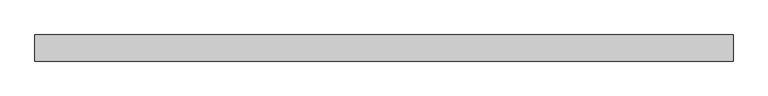
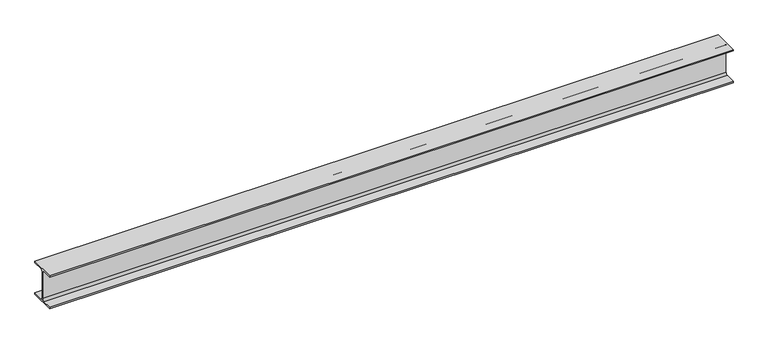
"""IFC4 building model written with IfcOpenShell, lengths in millimetres: beam geometry, 0912_Steel Framing_H-KSD3502 : H_SB_ASB_H-340x250x9x14."""

from ifc_helpers import new_model, si_unit, point, frame, frame_2d, origin, place, context, project, spatial, polyline, circle_curve, trimmed, segment, composite_curve, outline, extrude, source, transform, mapped, element, save


def beam_bd123048(model_context):
    return source(origin(), model_context, "Body", "SweptSolid", [
        extrude(outline(composite_curve([segment(polyline([(125.0, -156.0), (125.0, -170.0), (-125.0, -170.0), (-125.0, -156.0), (-24.5, -156.0)]), True, "CONTINUOUS"), segment(trimmed(circle_curve(frame_2d((-24.5, -136.0)), 20.0), [point((-24.5, -156.0))], [point((-4.5, -136.0))], True, "CARTESIAN"), True, "CONTINUOUS"), segment(polyline([(-4.5, -136.0), (-4.5, 136.0)]), True, "CONTINUOUS"), segment(trimmed(circle_curve(frame_2d((-24.5, 136.0)), 20.0), [point((-4.5, 136.0))], [point((-24.5, 156.0))], True, "CARTESIAN"), True, "CONTINUOUS"), segment(polyline([(-24.5, 156.0), (-125.0, 156.0), (-125.0, 170.0), (125.0, 170.0), (125.0, 156.0), (24.5, 156.0)]), True, "CONTINUOUS"), segment(trimmed(circle_curve(frame_2d((24.5, 136.0)), 20.0), [point((24.5, 156.0))], [point((4.5, 136.0))], True, "CARTESIAN"), True, "CONTINUOUS"), segment(polyline([(4.5, 136.0), (4.5, -136.0)]), True, "CONTINUOUS"), segment(trimmed(circle_curve(frame_2d((24.5, -136.0)), 20.0), [point((4.5, -136.0))], [point((24.5, -156.0))], True, "CARTESIAN"), True, "CONTINUOUS"), segment(polyline([(24.5, -156.0), (125.0, -156.0)]), True, "CONTINUOUS")], self_intersect=False)), frame((-3337.3, 0.0, 0.0), z_axis=(1.0, 0.0, 0.0), x_axis=(0.0, 1.0, 0.0)), (0.0, 0.0, 1.0), 6674.6),
    ])


if __name__ == "__main__":
    model = new_model("IFC4")
    model_context = context("Model", 3, world=origin())
    ifc_project = project(units=[si_unit("LENGTHUNIT", "METRE", prefix="MILLI")], contexts=[model_context])
    site = spatial("IfcSite", under=ifc_project)
    building = spatial("IfcBuilding", under=site)
    placement = place(None, origin())
    beam_shape = beam_bd123048(model_context)
    element("IfcBeam", 1, ObjectType="0912_Steel Framing_H-KSD3502 : H_SB_ASB_H-340x250x9x14", at=placement, inside=building, context=model_context, shape_type="MappedRepresentation", body=[
        mapped(beam_shape, transform((0.0, 0.0, 0.0), x_axis=(1.0, 0.0, 0.0), y_axis=(0.0, 1.0, 0.0), z_axis=(0.0, 0.0, 1.0))),
    ])
    save(model, "model.ifc")

# Revit data of these elements
# Type "0912_Steel Framing_H-KSD3502 : H_SB_ASB_H-340x250x9x14"
#   H_WM Code_1 = "S01AA002-00001 | Main Steel Structure Fabrication Work | Shelter/Building | Medium Steel - Standard (90KG/M>Weight≥30KG/M) | Material: (   )"
#   H_WM Code_2 = "S03AA028-00001 | Main Steel Structure Erection Work | Shelter/Building | Medium Steel (90KG/M>Weight≥30KG/M) | Material: (   )"
#   H_WM Code_3 = "S01AA010-00001 | Main Steel Structure Fabrication Work | Shelter/Building | Steel Painting/Coating | for Non-Fireproofed Steel Surface, Surface Preparation, Primer, Second & Final Coat | Material: (   )"
#   H_Q'ty Cal Type Tag = "SB-Q2"
#   Width = 25.0 cm
#   Web Thickness = 0.9 cm
#   Web Fillet = 2.0 cm
#   Warping Constant = 969000.0 cm⁶
#   W = 0
#   Torsional Moment of Inertia = 53.6551 cm⁴
#   Section Area = 101.5 cm²
#   Plastic Modulus weak axis = 447.0 cm³
#   Plastic Modulus strong axis = 1410.0 cm³
#   Perimeter = 1.63 m²/m
#   Nominal Weight = 79.70 kgf/m
#   Moment of Inertia weak axis = 3650.00 cm⁴
#   Moment of Inertia strong axis = 21700.00 cm⁴
#   Height = 34.0 cm
#   Flange Thickness = 1.4 cm
#   Elastic Modulus weak axis = 292.0 cm³
#   Elastic Modulus strong axis = 1280.0 cm³
#   Centroid Vertical = 17.0 cm
#   Centroid Horizontal = 12.5 cm
#   Ix = 217000000
#   Length [instance default] = 1.5240 m
#   Zx = 1410000
#   b = 0.2500 m
#   h = 0.3400 m
#   r = 0.0200 m
#   s = 0.0090 m
#   t = 0.0140 m
#   A = 0.01015 m²
#   Structural Material [instance default] = Steel, 45-345
#   Assembly Code = ""
# Element 1 (IfcBeam, "0912_Steel Framing_H-KSD3502 : H_SB_ASB_H-340x250x9x14")
#   Structural Material = none
# Materials
#   "Steel, 45-345": class "Metal", colour RGB 189 187 185, transparency 0, Description = "Steel 345 MPa", Cost = 0
